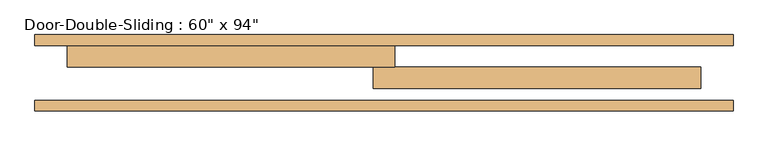
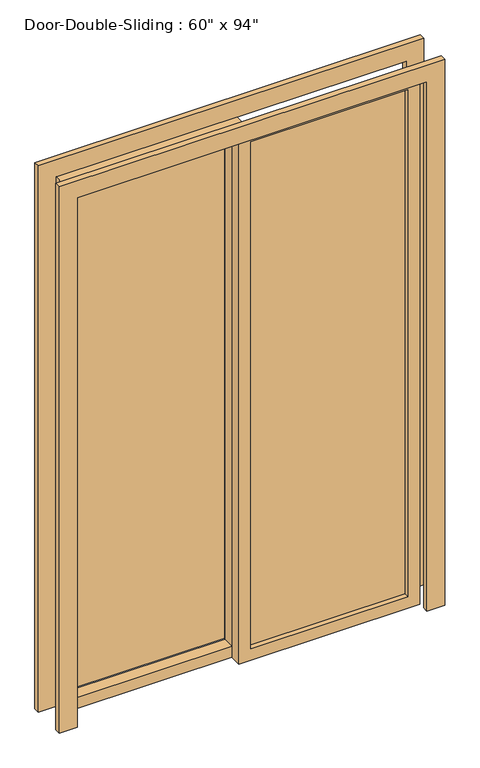
"""IFC4 building model written with IfcOpenShell, lengths in millimetres: door geometry."""

from ifc_helpers import new_model, si_unit, frame, origin, place, context, project, spatial, polyline, outline, extrude, source, transform, mapped, element, save


def door_dc317ca0(model_context):
    return source(origin(), model_context, "Body", "SweptSolid", [
        extrude(outline(polyline([(0.0, 826.2), (2476.2, 826.2), (2476.2, -826.2), (0.0, -826.2), (0.0, -750.0), (2400.0, -750.0), (2400.0, 750.0), (0.0, 750.0), (0.0, 826.2)])), frame((0.0, 192.0, 0.0), z_axis=(0.0, 1.0, 0.0), x_axis=(0.0, 0.0, 1.0)), (0.0, 0.0, 1.0), 25.4),
        extrude(outline(polyline([(0.0, -826.2), (0.0, -750.0), (2400.0, -750.0), (2400.0, 750.0), (0.0, 750.0), (0.0, 826.2), (2476.2, 826.2), (2476.2, -826.2), (0.0, -826.2)])), frame((0.0, 36.6, 0.0), z_axis=(0.0, 1.0, 0.0), x_axis=(0.0, 0.0, 1.0)), (0.0, 0.0, 1.0), 25.4),
        extrude(outline(polyline([(2400.0, 25.4), (2400.0, -750.0), (0.0, -750.0), (0.0, 25.4), (2400.0, 25.4)]), holes=[polyline([(2349.2, -25.4), (50.8, -25.4), (50.8, -699.2), (2349.2, -699.2), (2349.2, -25.4)])]), frame((0.0, 141.2, 0.0), z_axis=(0.0, 1.0, 0.0), x_axis=(0.0, 0.0, 1.0)), (0.0, 0.0, 1.0), 50.8),
        extrude(outline(polyline([(2400.0, -25.4), (0.0, -25.4), (0.0, 750.0), (2400.0, 750.0), (2400.0, -25.4)]), holes=[polyline([(2349.2, 25.4), (2349.2, 699.2), (50.8, 699.2), (50.8, 25.4), (2349.2, 25.4)])]), frame((0.0, 90.4, 0.0), z_axis=(0.0, 1.0, 0.0), x_axis=(0.0, 0.0, 1.0)), (0.0, 0.0, 1.0), 50.8),
        extrude(outline(polyline([(-25.4, 200.025), (-699.2, 200.025), (-699.2, 206.375), (-25.4, 206.375), (-25.4, 200.025)])), frame((0.0, 0.0, 50.8), z_axis=(0.0, 0.0, 1.0), x_axis=(1.0, 0.0, 0.0)), (0.0, 0.0, 1.0), 2298.4),
        extrude(outline(polyline([(25.4, 118.975), (699.2, 118.975), (699.2, 112.625), (25.4, 112.625), (25.4, 118.975)])), frame((0.0, 0.0, 50.8), z_axis=(0.0, 0.0, 1.0), x_axis=(1.0, 0.0, 0.0)), (0.0, 0.0, 1.0), 2298.4),
    ])


if __name__ == "__main__":
    model = new_model("IFC4")
    model_context = context("Model", 3, world=origin())
    ifc_project = project(units=[si_unit("LENGTHUNIT", "METRE", prefix="MILLI")], contexts=[model_context])
    site = spatial("IfcSite", under=ifc_project)
    building = spatial("IfcBuilding", under=site)
    placement = place(None, origin())
    door_shape = door_dc317ca0(model_context)
    element("IfcDoor", 1, ObjectType="Door-Double-Sliding : 60\" x 94\"", at=placement, inside=building, context=model_context, shape_type="MappedRepresentation", body=[
        mapped(door_shape, transform((0.0, 0.0, 0.0), x_axis=(1.0, 0.0, 0.0), y_axis=(0.0, 1.0, 0.0), z_axis=(0.0, 0.0, 1.0))),
    ])
    save(model, "model.ifc")

# Revit data of these elements
# Type "Door-Double-Sliding : 60\" x 94\""
#   Type Mark = "62"
#   Construction Type Id = "opn-d45"
#   Assembly Code = "C1020"
#   Analytic Construction = "Wood frame, double glass door "
#   Thickness = 50.8 mm
#   Thermal Resistance (R) = 0.31964 (m²·K)/W
#   Heat Transfer Coefficient (U) = 3.12872 W/(m²·K)
#   Height = 2400 mm
#   Rail Width = 50.8 mm
#   Stiles = 50.8 mm
#   Trim Projection Ext = 25.4 mm
#   Trim Projection Int = 25.4 mm
#   Trim Width = 76.2 mm
#   Width = 1500 mm
#   Define Thermal Properties by = 1
#   Glazing = Glass
#   Panel Material = Wood - Birch - Solid Stained Light Low Gloss
#   Trim Material = Paint - Sienna
#   Visual Light Transmittance = 0
#   Solar Heat Gain Coefficient = 0
#   Function = (empty or 0)
#   Wall Closure = (empty or 0)
# Element 1 (IfcDoor, "Door-Double-Sliding : 60\" x 94\"")
#   Materials on its faces: "Paint - Sienna", "Wood - Birch - Solid Stained Light Low Gloss", "Glass"
# Materials
#   "Glass": class "Glass", colour RGB 0 128 192, transparency 0.9, Description = "Soda Lime Glass", Cost = 0
#   "Wood - Birch - Solid Stained Light Low Gloss": class "Wood", colour RGB 210 159 95, transparency 0, Cost = 0
#   "Paint - Sienna": class "Miscellaneous", colour RGB 118 70 51, transparency 0, Cost = 0
